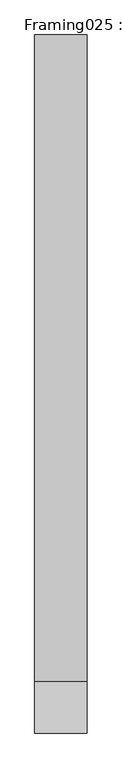
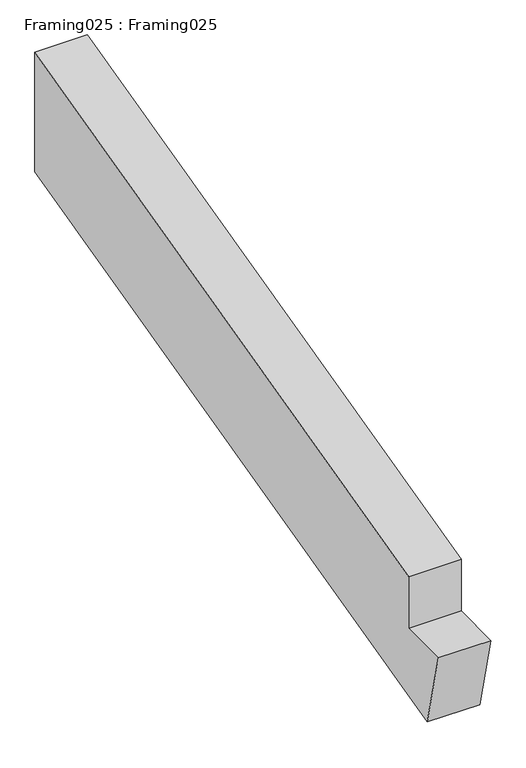
"""IFC4 building model written with IfcOpenShell, lengths in millimetres: proxy geometry, Framing025 : Framing025."""

from ifc_helpers import new_model, si_unit, frame, origin, place, context, project, spatial, polyline, outline, extrude, source, transform, mapped, element, save


def framing025_framing025_fdaa2fb1(model_context):
    return source(origin(), model_context, "Body", "SweptSolid", [
        extrude(outline(polyline([(-5374.9745897, 42642.0307603), (-5224.4076049, 42642.0307603), (-5224.4076049, 42800.8143799), (-3344.6566162, 43270.717426), (-3344.6566162, 42903.8818003), (-5318.455674, 42411.3663805), (-5374.9745897, 42642.0307603)])), frame((12534.9, 0.0, 0.0), z_axis=(1.0, 0.0, 0.0), x_axis=(0.0, 1.0, 0.0)), (0.0, 0.0, 1.0), 152.4),
    ])


if __name__ == "__main__":
    model = new_model("IFC4")
    model_context = context("Model", 3, world=origin())
    ifc_project = project(units=[si_unit("LENGTHUNIT", "METRE", prefix="MILLI")], contexts=[model_context])
    site = spatial("IfcSite", under=ifc_project)
    building = spatial("IfcBuilding", under=site)
    placement = place(None, origin())
    framing025_framing025_shape = framing025_framing025_fdaa2fb1(model_context)
    element("IfcBuildingElementProxy", 1, Name="Framing025 : Framing025", ObjectType="Framing025 : Framing025", at=placement, inside=building, context=model_context, shape_type="MappedRepresentation", body=[
        mapped(framing025_framing025_shape, transform((0.0, 0.0, 0.0), x_axis=(1.0, 0.0, 0.0), y_axis=(0.0, 1.0, 0.0), z_axis=(0.0, 0.0, 1.0))),
    ])
    save(model, "model.ifc")

# Revit data of these elements
# Type "Framing025 : Framing025"
#   NameOverride = "Framing025"
# Element 1 (IfcBuildingElementProxy, "Framing025 : Framing025")
#   Materials on its faces: "WOOD FRAMING (SEE STRUCT DWGS)"
# Materials
#   "WOOD FRAMING (SEE STRUCT DWGS)": class "Unassigned", colour RGB 224 188 168, transparency 0, Cost = 0
